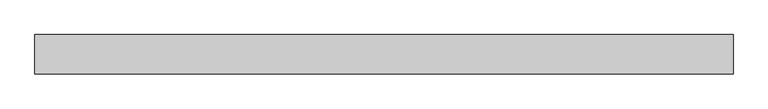
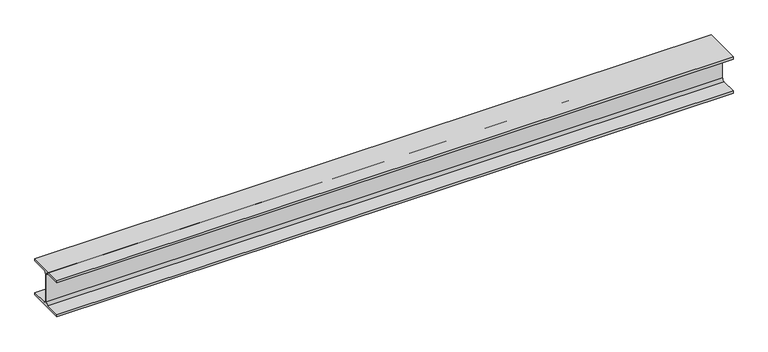
"""IFC4 building model written with IfcOpenShell, lengths in millimetres: beam geometry, 0912_Steel Framing_H-KSD3502 : H_SB_ASB_H-200x200x8x12."""

import ifcopenshell
import ifcopenshell.guid

model = None  # the IFC model being written
_history = None  # IfcOwnerHistory: only IFC2X3 demands one
_inside = {}  # id of a spatial element -> (the spatial element, [elements in it])
_under = {}  # id of a project, library or spatial element -> (it, [spatial elements below it])
_declared = {}  # id of a project -> (the project, [libraries it declares])
_typed = {}  # id of a type object -> (the type object, [elements of that type])
_made_of = {}  # id of a material, layer set ... -> (it, [elements and type objects made of it])


def new_model(schema):
    """Start an empty IFC model of exactly this schema.

    Asked for "IFC4X3", IfcOpenShell would pick the latest addendum, in which some entities
    have other attributes; the version numbers below select the first issue.
    IFC2X3 requires an IfcOwnerHistory on every rooted entity: one is made here for all.
    """
    global model, _history
    if schema == "IFC4X3":
        model = ifcopenshell.file(schema_version=(4, 3, 0, 0))
    else:
        model = ifcopenshell.file(schema=schema)
    _inside.clear()
    _under.clear()
    _declared.clear()
    _typed.clear()
    _made_of.clear()
    _history = None
    if model.schema == "IFC2X3":
        org = make("IfcOrganization", Name="unknown")
        user = make(
            "IfcPersonAndOrganization",
            ThePerson=make("IfcPerson", FamilyName="unknown"),
            TheOrganization=org,
        )
        app = make(
            "IfcApplication",
            ApplicationDeveloper=org,
            Version="unknown",
            ApplicationFullName="unknown",
            ApplicationIdentifier="unknown",
        )
        _history = make(
            "IfcOwnerHistory",
            OwningUser=user,
            OwningApplication=app,
            ChangeAction="ADDED",
            CreationDate=0,
        )
    return model


def make(cls, **values):
    """One entity of the class cls with the attributes given. An attribute that is None is left unset."""
    return model.create_entity(
        cls, **{name: value for name, value in values.items() if value is not None}
    )


def rooted(cls, **values):
    """An entity with a GlobalId (a new one), such as an element, a storey or a relation."""
    return make(cls, GlobalId=ifcopenshell.guid.new(), OwnerHistory=_history, **values)


def si_unit(unit_type, name, prefix=None):
    """IfcSIUnit, for example si_unit("LENGTHUNIT", "METRE", prefix="MILLI")."""
    return make("IfcSIUnit", UnitType=unit_type, Prefix=prefix, Name=name)


def assignment(units):
    """IfcUnitAssignment: the units of a project."""
    return None if units is None else make("IfcUnitAssignment", Units=units)


def point(xyz):
    """IfcCartesianPoint."""
    return None if xyz is None else make("IfcCartesianPoint", Coordinates=xyz)


def direction(xyz):
    """IfcDirection."""
    return None if xyz is None else make("IfcDirection", DirectionRatios=xyz)


def frame(location, z_axis=None, x_axis=None):
    """IfcAxis2Placement3D, a coordinate frame: its origin and axes. An axis left out is left unset."""
    return make(
        "IfcAxis2Placement3D",
        Location=point(location),
        Axis=direction(z_axis),
        RefDirection=direction(x_axis),
    )


def frame_2d(location, x_axis=None):
    """IfcAxis2Placement2D, a coordinate frame in the plane: its origin and x axis."""
    return make(
        "IfcAxis2Placement2D", Location=point(location), RefDirection=direction(x_axis)
    )


def origin():
    """The frame at (0, 0, 0) with its axes left unset."""
    return frame((0.0, 0.0, 0.0))


def place(relative_to, where):
    """IfcLocalPlacement: puts the frame where relative to a parent placement (None: the world)."""
    return make(
        "IfcLocalPlacement", PlacementRelTo=relative_to, RelativePlacement=where
    )


def context(
    kind, dimensions, precision=None, world=None, true_north=None, identifier=None
):
    """IfcGeometricRepresentationContext, for example the 3D "Model" context."""
    return make(
        "IfcGeometricRepresentationContext",
        ContextIdentifier=identifier,
        ContextType=kind,
        CoordinateSpaceDimension=dimensions,
        Precision=precision,
        WorldCoordinateSystem=world,
        TrueNorth=true_north,
    )


def project(units=None, contexts=None):
    """IfcProject with its units and contexts."""
    return rooted(
        "IfcProject",
        Name="project",
        RepresentationContexts=contexts,
        UnitsInContext=assignment(units),
    )


def spatial(cls, under=None, at=None, **own):
    """A site, building, storey or space (cls), placed at a placement, below another one or the project."""
    s = rooted(cls, ObjectPlacement=at, **own)
    if under is not None:
        _under.setdefault(under.id(), (under, []))[1].append(s)
    return s


def polyline(points):
    """IfcPolyline through the points."""
    return make("IfcPolyline", Points=[point(p) for p in points])


def circle_curve(where, radius):
    """IfcCircle in the frame where."""
    return make("IfcCircle", Position=where, Radius=radius)


def trimmed(basis, trim1, trim2, sense, master):
    """IfcTrimmedCurve: the piece of a basis curve between two trims."""
    return make(
        "IfcTrimmedCurve",
        BasisCurve=basis,
        Trim1=trim1,
        Trim2=trim2,
        SenseAgreement=sense,
        MasterRepresentation=master,
    )


def segment(curve, same_sense, transition):
    """IfcCompositeCurveSegment."""
    return make(
        "IfcCompositeCurveSegment",
        Transition=transition,
        SameSense=same_sense,
        ParentCurve=curve,
    )


def composite_curve(segments, self_intersect=None):
    """IfcCompositeCurve: segments joined end to end."""
    return make("IfcCompositeCurve", Segments=segments, SelfIntersect=self_intersect)


def outline(outer, holes=None, kind="AREA"):
    """IfcArbitraryClosedProfileDef: a profile drawn as a closed curve; with holes, ...WithVoids."""
    if holes is None:
        return make("IfcArbitraryClosedProfileDef", ProfileType=kind, OuterCurve=outer)
    return make(
        "IfcArbitraryProfileDefWithVoids",
        ProfileType=kind,
        OuterCurve=outer,
        InnerCurves=holes,
    )


def extrude(swept, where, along, depth):
    """IfcExtrudedAreaSolid: the profile swept, set in the frame where, extruded along a direction by depth."""
    return make(
        "IfcExtrudedAreaSolid",
        SweptArea=swept,
        Position=where,
        ExtrudedDirection=direction(along),
        Depth=depth,
    )


def shape(context_of_items, identifier, shape_type, items):
    """IfcShapeRepresentation: the items that make up one representation, for example the "Body"."""
    return make(
        "IfcShapeRepresentation",
        ContextOfItems=context_of_items,
        RepresentationIdentifier=identifier,
        RepresentationType=shape_type,
        Items=items,
    )


def source(mapping_origin, context_of_items, identifier, shape_type, items):
    """IfcRepresentationMap: a shape defined once, which mapped items show again and again."""
    return make(
        "IfcRepresentationMap",
        MappingOrigin=mapping_origin,
        MappedRepresentation=shape(context_of_items, identifier, shape_type, items),
    )


def transform(
    local_origin,
    x_axis=None,
    y_axis=None,
    z_axis=None,
    scale=None,
    scale2=None,
    scale3=None,
    uniform=True,
):
    """IfcCartesianTransformationOperator3D, or its non-uniform kind. x_axis, y_axis, z_axis: its Axis1, 2, 3."""
    if uniform:
        return make(
            "IfcCartesianTransformationOperator3D",
            Axis1=direction(x_axis),
            Axis2=direction(y_axis),
            LocalOrigin=point(local_origin),
            Scale=scale,
            Axis3=direction(z_axis),
        )
    return make(
        "IfcCartesianTransformationOperator3DnonUniform",
        Axis1=direction(x_axis),
        Axis2=direction(y_axis),
        LocalOrigin=point(local_origin),
        Scale=scale,
        Axis3=direction(z_axis),
        Scale2=scale2,
        Scale3=scale3,
    )


def mapped(mapping_source, mapping_target):
    """IfcMappedItem: shows the shape of a source again, moved by a transform."""
    return make(
        "IfcMappedItem", MappingSource=mapping_source, MappingTarget=mapping_target
    )


def made_of(thing, what):
    """Note that an element or type object is made of a material, layer set ...; save() writes the relation."""
    if what is not None:
        _made_of.setdefault(what.id(), (what, []))[1].append(thing)
    return thing


def element(
    cls,
    number,
    at=None,
    inside=None,
    cuts=None,
    type_object=None,
    material=None,
    context=None,
    identifier="Body",
    shape_type=None,
    held_by="IfcProductDefinitionShape",
    body=None,
    shapes=None,
    **own,
):
    """One element of the class cls, such as IfcWall. Its Tag is "e" and its number.

    at: its placement. inside: the storey or other place that contains it. cuts: it is an
    opening in that element (IfcRelVoidsElement). A single representation is given by context,
    identifier, shape_type and body (its items); several are given by shapes. held_by: the class
    of the entity that holds the representations. save() writes the other relations.
    """
    e = rooted(cls, Tag="e%d" % number, ObjectPlacement=at, **own)
    if body is not None:
        shapes = [shape(context, identifier, shape_type, body)]
    if shapes is not None:
        e.Representation = make(held_by, Representations=shapes)
    if inside is not None:
        _inside.setdefault(inside.id(), (inside, []))[1].append(e)
    if cuts is not None:
        rooted(
            "IfcRelVoidsElement", RelatingBuildingElement=cuts, RelatedOpeningElement=e
        )
    if type_object is not None:
        _typed.setdefault(type_object.id(), (type_object, []))[1].append(e)
    return made_of(e, material)


def aggregate(whole, parts):
    """IfcRelAggregates: a whole, such as a stair, and the parts it consists of."""
    return rooted("IfcRelAggregates", RelatingObject=whole, RelatedObjects=parts)


def save(model, path):
    """Write the relations noted so far, then the file.

    IfcRelAggregates (storeys below a building ...), IfcRelContainedInSpatialStructure (elements
    in a storey), IfcRelDefinesByType, IfcRelAssociatesMaterial and IfcRelDeclares: one each for
    every whole, place, type object, material and project.
    """
    for whole, parts in _under.values():
        aggregate(whole, parts)
    for where, things in _inside.values():
        rooted(
            "IfcRelContainedInSpatialStructure",
            RelatedElements=things,
            RelatingStructure=where,
        )
    for kind, things in _typed.values():
        rooted("IfcRelDefinesByType", RelatedObjects=things, RelatingType=kind)
    for what, things in _made_of.values():
        rooted("IfcRelAssociatesMaterial", RelatedObjects=things, RelatingMaterial=what)
    for by, libraries in _declared.values():
        rooted("IfcRelDeclares", RelatingContext=by, RelatedDefinitions=libraries)
    model.write(path)


def beam_e80e70f2(model_context):
    return source(origin(), model_context, "Body", "SweptSolid", [
        extrude(outline(composite_curve([segment(polyline([(100.0, -88.0), (100.0, -100.0), (-100.0, -100.0), (-100.0, -88.0), (-17.0, -88.0)]), True, "CONTINUOUS"), segment(trimmed(circle_curve(frame_2d((-17.0, -75.0)), 13.0), [point((-17.0, -88.0))], [point((-4.0, -75.0))], True, "CARTESIAN"), True, "CONTINUOUS"), segment(polyline([(-4.0, -75.0), (-4.0, 75.0)]), True, "CONTINUOUS"), segment(trimmed(circle_curve(frame_2d((-17.0, 75.0)), 13.0), [point((-4.0, 75.0))], [point((-17.0, 88.0))], True, "CARTESIAN"), True, "CONTINUOUS"), segment(polyline([(-17.0, 88.0), (-100.0, 88.0), (-100.0, 100.0), (100.0, 100.0), (100.0, 88.0), (17.0, 88.0)]), True, "CONTINUOUS"), segment(trimmed(circle_curve(frame_2d((17.0, 75.0)), 13.0), [point((17.0, 88.0))], [point((4.0, 75.0))], True, "CARTESIAN"), True, "CONTINUOUS"), segment(polyline([(4.0, 75.0), (4.0, -75.0)]), True, "CONTINUOUS"), segment(trimmed(circle_curve(frame_2d((17.0, -75.0)), 13.0), [point((4.0, -75.0))], [point((17.0, -88.0))], True, "CARTESIAN"), True, "CONTINUOUS"), segment(polyline([(17.0, -88.0), (100.0, -88.0)]), True, "CONTINUOUS")], self_intersect=False)), frame((-1725.502423, 0.0, 0.0), z_axis=(1.0, 0.0, 0.0), x_axis=(0.0, 1.0, 0.0)), (0.0, 0.0, 1.0), 3536.3433078),
    ])


if __name__ == "__main__":
    model = new_model("IFC4")
    model_context = context("Model", 3, world=origin())
    ifc_project = project(units=[si_unit("LENGTHUNIT", "METRE", prefix="MILLI")], contexts=[model_context])
    site = spatial("IfcSite", under=ifc_project)
    building = spatial("IfcBuilding", under=site)
    placement = place(None, origin())
    beam_shape = beam_e80e70f2(model_context)
    element("IfcBeam", 1, ObjectType="0912_Steel Framing_H-KSD3502 : H_SB_ASB_H-200x200x8x12", at=placement, inside=building, context=model_context, shape_type="MappedRepresentation", body=[
        mapped(beam_shape, transform((0.0, 0.0, 0.0), x_axis=(1.0, 0.0, 0.0), y_axis=(0.0, 1.0, 0.0), z_axis=(0.0, 0.0, 1.0))),
    ])
    save(model, "model.ifc")

# Revit data of these elements
# Type "0912_Steel Framing_H-KSD3502 : H_SB_ASB_H-200x200x8x12"
#   H_WM Code_1 = "S01AA002-00001 | Main Steel Structure Fabrication Work | Shelter/Building | Medium Steel - Standard (90KG/M>Weight≥30KG/M) | Material: (   )"
#   H_WM Code_2 = "S03AA028-00001 | Main Steel Structure Erection Work | Shelter/Building | Medium Steel (90KG/M>Weight≥30KG/M) | Material: (   )"
#   H_WM Code_3 = "S01AA010-00001 | Main Steel Structure Fabrication Work | Shelter/Building | Steel Painting/Coating | for Non-Fireproofed Steel Surface, Surface Preparation, Primer, Second & Final Coat | Material: (   )"
#   H_Q'ty Cal Type Tag = "SB-Q2"
#   Width = 20.0 cm
#   Web Thickness = 0.8 cm
#   Web Fillet = 1.3 cm
#   Warping Constant = 141000.0 cm⁶
#   W = 0
#   Torsional Moment of Inertia = 26.2485 cm⁴
#   Section Area = 63.53 cm²
#   Plastic Modulus weak axis = 244.0 cm³
#   Plastic Modulus strong axis = 525.0 cm³
#   Perimeter = 1.16 m²/m
#   Nominal Weight = 49.90 kgf/m
#   Moment of Inertia weak axis = 1600.00 cm⁴
#   Moment of Inertia strong axis = 4720.00 cm⁴
#   Height = 20.0 cm
#   Flange Thickness = 1.2 cm
#   Elastic Modulus weak axis = 160.0 cm³
#   Elastic Modulus strong axis = 472.0 cm³
#   Centroid Vertical = 10.0 cm
#   Centroid Horizontal = 10.0 cm
#   Ix = 47200000
#   Length [instance default] = 1.5240 m
#   Zx = 525000
#   b = 0.2000 m
#   h = 0.2000 m
#   r = 0.0130 m
#   s = 0.0080 m
#   t = 0.0120 m
#   A = 0.006353 m²
#   Structural Material [instance default] = Steel, 45-345
#   Assembly Code = ""
# Element 1 (IfcBeam, "0912_Steel Framing_H-KSD3502 : H_SB_ASB_H-200x200x8x12")
#   Structural Material = none
# Materials
#   "Steel, 45-345": class "Metal", colour RGB 189 187 185, transparency 0, Description = "Steel 345 MPa", Cost = 0
